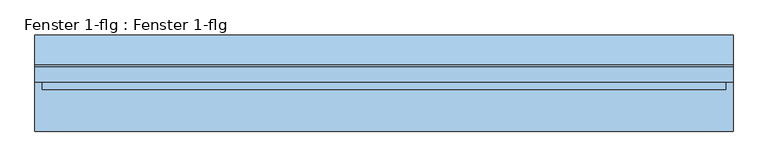
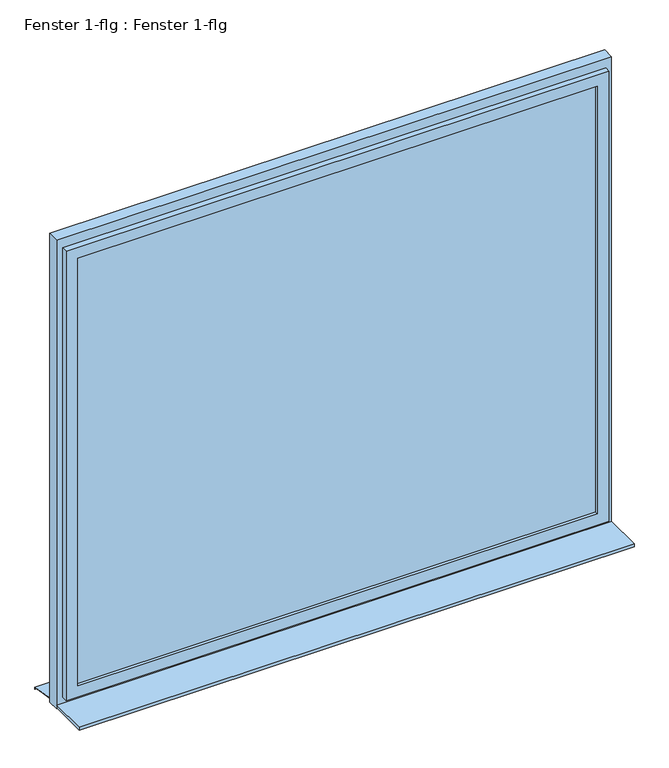
"""IFC4 building model written with IfcOpenShell, lengths in millimetres: window geometry, Fenster 1-flg : Fenster 1-flg."""

from ifc_helpers import new_model, si_unit, frame, origin, place, context, project, spatial, polyline, outline, extrude, faceted_brep, source, transform, mapped, element, save


def fenster_1_flg_fenster_1_flg_fbf7811f(model_context):
    return source(origin(), model_context, "Body", "SolidModel", [
        extrude(outline(polyline([(3500.0, 1400.0), (3500.0, -1400.0), (1000.0, -1400.0), (1000.0, 1400.0), (3500.0, 1400.0)]), holes=[polyline([(3420.0, 1340.0), (1080.0, 1340.0), (1080.0, -1340.0), (3420.0, -1340.0), (3420.0, 1340.0)])]), frame((0.0, 3.5, 0.0), z_axis=(0.0, 1.0, 0.0), x_axis=(0.0, 0.0, 1.0)), (0.0, 0.0, 1.0), 60.0),
        faceted_brep([(1370.0, 3.5, 3450.0), (1370.0, -26.5, 3450.0), (1370.0, -26.5, 1050.0), (1370.0, 3.5, 1050.0), (-1370.0, -26.5, 3450.0), (-1370.0, -26.5, 1050.0), (1310.0, -26.5, 1110.0), (-1310.0, -26.5, 1110.0), (-1310.0, -26.5, 3390.0), (1310.0, -26.5, 3390.0), (-1370.0, 3.5, 1050.0), (-1370.0, 3.5, 3450.0), (1340.0, 3.5, 3420.0), (-1340.0, 3.5, 3420.0), (-1340.0, 3.5, 1080.0), (1340.0, 3.5, 1080.0), (1340.0, 33.5, 3420.0), (1340.0, 33.5, 1080.0), (-1340.0, 33.5, 1080.0), (-1340.0, 33.5, 3420.0), (1310.0, 33.5, 3390.0), (-1310.0, 33.5, 3390.0), (-1310.0, 33.5, 1110.0), (1310.0, 33.5, 1110.0)], [[[0, 1, 2, 3]], [[1, 4, 5, 2], [6, 7, 8, 9]], [[3, 2, 5, 10]], [[3, 10, 11, 0], [12, 13, 14, 15]], [[16, 12, 15, 17]], [[17, 15, 14, 18]], [[17, 18, 19, 16], [20, 21, 22, 23]], [[9, 20, 23, 6]], [[6, 23, 22, 7]], [[10, 5, 4, 11]], [[18, 14, 13, 19]], [[7, 22, 21, 8]], [[11, 4, 1, 0]], [[19, 13, 12, 16]], [[8, 21, 20, 9]]]),
        extrude(outline(polyline([(-1400.0, -193.5), (-1400.0, 3.5), (1400.0, 3.5), (1400.0, -193.5), (-1400.0, -193.5)])), frame((0.0, 0.0, 1005.0), z_axis=(0.0, 0.0, 1.0), x_axis=(1.0, 0.0, 0.0)), (0.0, 0.0, 1.0), 15.0),
        extrude(outline(polyline([(73.5221543, 1020.0), (193.5, 1000.0), (193.5, 990.0), (191.5, 990.0), (191.5, 998.3604634), (73.3240723, 1018.0), (63.5, 1018.0), (63.5, 1020.0), (73.5221543, 1020.0)])), frame((-1400.0, 0.0, 0.0), z_axis=(1.0, 0.0, 0.0), x_axis=(0.0, 1.0, 0.0)), (0.0, 0.0, 1.0), 2800.0),
        extrude(outline(polyline([(1310.0, -11.5), (-1310.0, -11.5), (-1310.0, 18.5), (1310.0, 18.5), (1310.0, -11.5)])), frame((0.0, 0.0, 1110.0), z_axis=(0.0, 0.0, 1.0), x_axis=(1.0, 0.0, 0.0)), (0.0, 0.0, 1.0), 2280.0),
    ])


if __name__ == "__main__":
    model = new_model("IFC4")
    model_context = context("Model", 3, world=origin())
    ifc_project = project(units=[si_unit("LENGTHUNIT", "METRE", prefix="MILLI")], contexts=[model_context])
    site = spatial("IfcSite", under=ifc_project)
    building = spatial("IfcBuilding", under=site)
    placement = place(None, origin())
    fenster_1_flg_fenster_1_flg_shape = fenster_1_flg_fenster_1_flg_fbf7811f(model_context)
    element("IfcWindow", 1, ObjectType="Fenster 1-flg : Fenster 1-flg", at=placement, inside=building, context=model_context, shape_type="MappedRepresentation", body=[
        mapped(fenster_1_flg_fenster_1_flg_shape, transform((0.0, 0.0, 0.0), x_axis=(1.0, 0.0, 0.0), y_axis=(0.0, 1.0, 0.0), z_axis=(0.0, 0.0, 1.0))),
    ])
    save(model, "model.ifc")

# Revit data of these elements
# Project information
#   Project Issue Date = "Ausgabedatum"
#   Project Status = "Projektstatus"
#   Client Name = "Besitzer"
#   Project Address = "Geben Sie die Adresse hier ein"
#   Project Name = "Projektname"
#   Project Number = "Projektnummer"
# Type "Fenster 1-flg : Fenster 1-flg"
#   Type Mark = "45"
#   Operation = "SinglePanel"
#   Construction Type Id = "RGDPK6R"
#   Keynote = "16.05.01"
#   Analytic Construction = "Low-E double glazing (1/4 in + 1/4 in)"
#   Visual Light Transmittance = 0.76
#   Thermal Resistance (R) = 0.179801 (m²·K)/W
#   Solar Heat Gain Coefficient = 0.65
#   Rough Width = 2800 mm
#   Rough Height = 2500 mm
#   Heat Transfer Coefficient (U) = 2.1030 W/(m²·K)
#   Rahmentiefe = 60 mm
#   Rahmenhöhe unten = 80 mm
#   Rahmenhöhe oben = 80 mm
#   Rahmenbreite = 60 mm
#   Height = 2500 mm
#   Flügeltiefe = 60 mm
#   Flügelbreite = 60 mm
#   Einbautiefe (von außen) [instance default] = 100 mm
#   Width = 2800 mm
#   Klappflügel [instance default] = no
#   Kippflügel [instance default] = yes
#   Öffnungsrichtung in Draufsicht anzeigen [instance default] = no
#   Drehflügel [instance default] = yes
#   Rahmen [instance default] = none
#   Glas [instance default] = none
#   Lüftungsöffnung [instance default] = none
#   Fensterbank innen [instance default] = none
#   Fensterbank außen [instance default] = none
#   Wall Closure = (empty or 0)
# Element 1 (IfcWindow, "Fenster 1-flg : Fenster 1-flg")
#   Materials on its faces: "Fenster - Kunststoff weiß", "Farbe Grau", "Glas", "Farbe Weiss", "Fenster - Holz"
# Materials
#   "Fenster - Kunststoff weiß": class "Kunststoff", colour RGB 249 249 249, transparency 0
#   "Farbe Grau": class "Generic", colour RGB 85 85 85, transparency 0, Cost = 0
#   "Glas": class "Glas", colour RGB 0 128 192, transparency 0.75, Description = "Kalknatronglas", Cost = 0
#   "Farbe Weiss": class "Generic", colour RGB 255 255 255, transparency 0, Cost = 0
#   "Fenster - Holz": class "Holz", colour RGB 216 135 75, transparency 0
